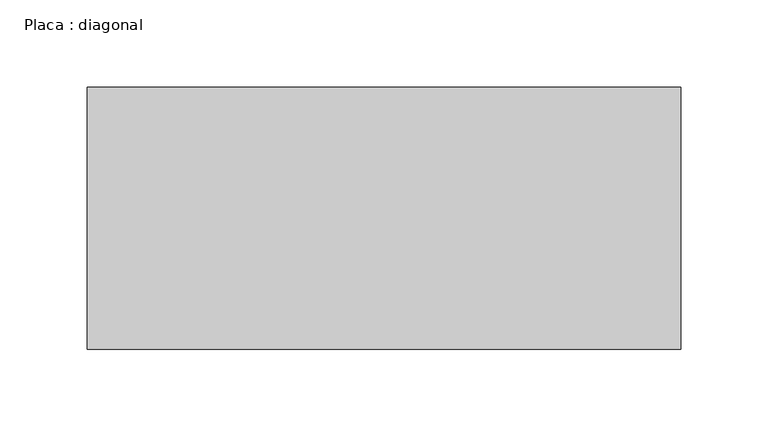
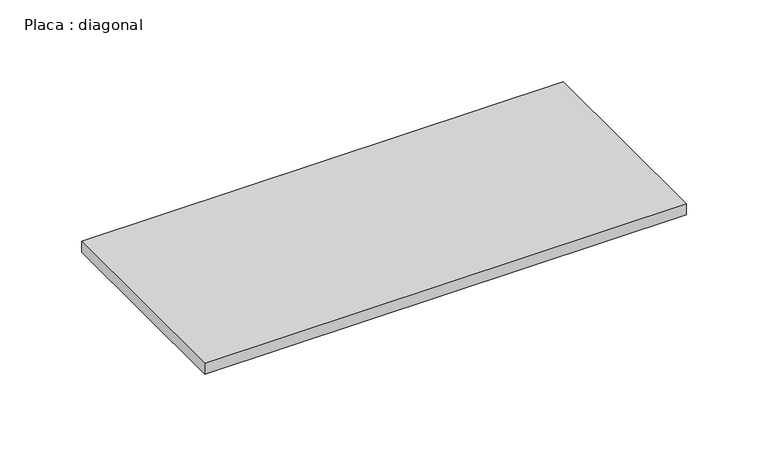
"""IFC4 building model written with IfcOpenShell, lengths in millimetres: beam geometry, Placa : diagonal."""

from ifc_helpers import new_model, si_unit, frame, origin, place, context, project, spatial, polyline, outline, extrude, source, transform, mapped, element, save


def placa_diagonal_c6130ff1(model_context):
    return source(origin(), model_context, "Body", "SweptSolid", [
        extrude(outline(polyline([(169.7794224, 75.0), (169.7794224, -75.0), (-169.7794224, -75.0), (-169.7794224, 75.0), (169.7794224, 75.0)])), frame((0.0, 0.0, -4.0), z_axis=(0.0, 0.0, 1.0), x_axis=(1.0, 0.0, 0.0)), (0.0, 0.0, 1.0), 8.0),
    ])


if __name__ == "__main__":
    model = new_model("IFC4")
    model_context = context("Model", 3, world=origin())
    ifc_project = project(units=[si_unit("LENGTHUNIT", "METRE", prefix="MILLI")], contexts=[model_context])
    site = spatial("IfcSite", under=ifc_project)
    building = spatial("IfcBuilding", under=site)
    placement = place(None, origin())
    placa_diagonal_shape = placa_diagonal_c6130ff1(model_context)
    element("IfcBeam", 1, ObjectType="Placa : diagonal", at=placement, inside=building, context=model_context, shape_type="MappedRepresentation", body=[
        mapped(placa_diagonal_shape, transform((0.0, 0.0, 0.0), x_axis=(1.0, 0.0, 0.0), y_axis=(0.0, 1.0, 0.0), z_axis=(0.0, 0.0, 1.0))),
    ])
    save(model, "model.ifc")

# Revit data of these elements
# Type "Placa : diagonal"
#   W = 0
#   Length [instance default] = 1.50 m
#   b = 0.15 m
#   d = 0.008 m
#   A = 0 m²
#   Structural Material [instance default] = Aço, 45-345
# Element 1 (IfcBeam, "Placa : diagonal")
#   Materials on its faces: "Aço, 45-345"
# Materials
#   "Aço, 45-345": class "Metal", colour RGB 247 247 247, transparency 0, Description = "Aço 345 MPa", Cost = 0
